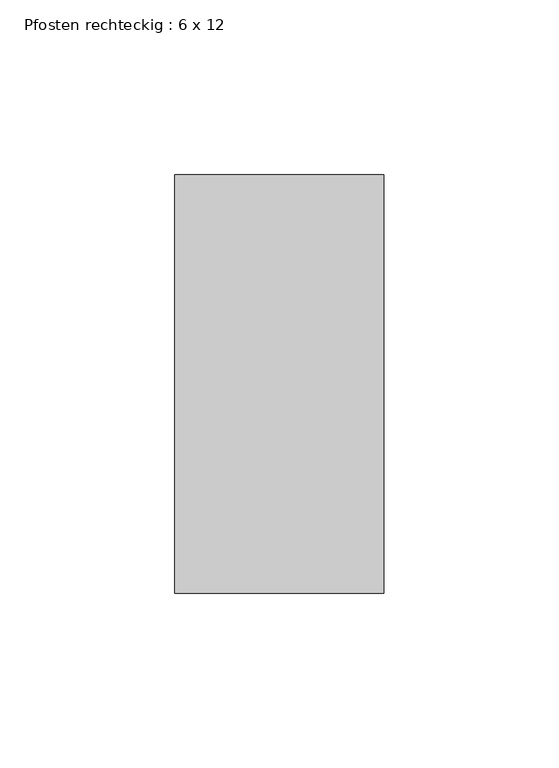
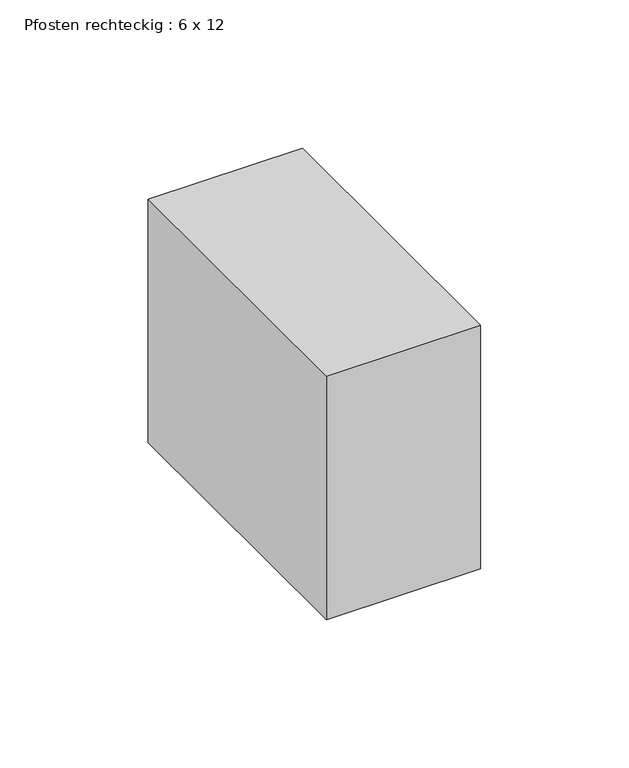
"""IFC4 building model written with IfcOpenShell, lengths in millimetres: member geometry, Pfosten rechteckig : 6 x 12."""

from ifc_helpers import new_model, si_unit, frame, origin, place, context, project, spatial, polyline, outline, extrude, source, transform, mapped, element, save


def pfosten_rechteckig_6_x_12_fc4c2c82(model_context):
    return source(origin(), model_context, "Body", "SweptSolid", [
        extrude(outline(polyline([(0.0, 60.0), (0.0, -60.0), (-60.0, -60.0), (-60.0, 60.0), (0.0, 60.0)])), frame((0.0, 0.0, -100.0), z_axis=(0.0, 0.0, 1.0), x_axis=(1.0, 0.0, 0.0)), (0.0, 0.0, 1.0), 100.0),
    ])


if __name__ == "__main__":
    model = new_model("IFC4")
    model_context = context("Model", 3, world=origin())
    ifc_project = project(units=[si_unit("LENGTHUNIT", "METRE", prefix="MILLI")], contexts=[model_context])
    site = spatial("IfcSite", under=ifc_project)
    building = spatial("IfcBuilding", under=site)
    placement = place(None, origin())
    pfosten_rechteckig_6_x_12_shape = pfosten_rechteckig_6_x_12_fc4c2c82(model_context)
    element("IfcMember", 1, ObjectType="Pfosten rechteckig : 6 x 12", at=placement, inside=building, context=model_context, shape_type="MappedRepresentation", body=[
        mapped(pfosten_rechteckig_6_x_12_shape, transform((0.0, 0.0, 0.0), x_axis=(1.0, 0.0, 0.0), y_axis=(0.0, 1.0, 0.0), z_axis=(0.0, 0.0, 1.0))),
    ])
    save(model, "model.ifc")

# Revit data of these elements
# Type "Pfosten rechteckig : 6 x 12"
#   built-in parameter 1007304 = 0.393701 (stored number, unit not read)
#   built-in parameter 1007301 = 0.0984252 (stored number, unit not read)
#   built-in parameter 1007300 = 0.0984252 (stored number, unit not read)
# Element 1 (IfcMember, "Pfosten rechteckig : 6 x 12")
#   Materials on its faces: "Metall - verzinkt"
# Materials
#   "Metall - verzinkt": class "Allgemeines", colour RGB 200 200 200, transparency 0, Cost = 0
